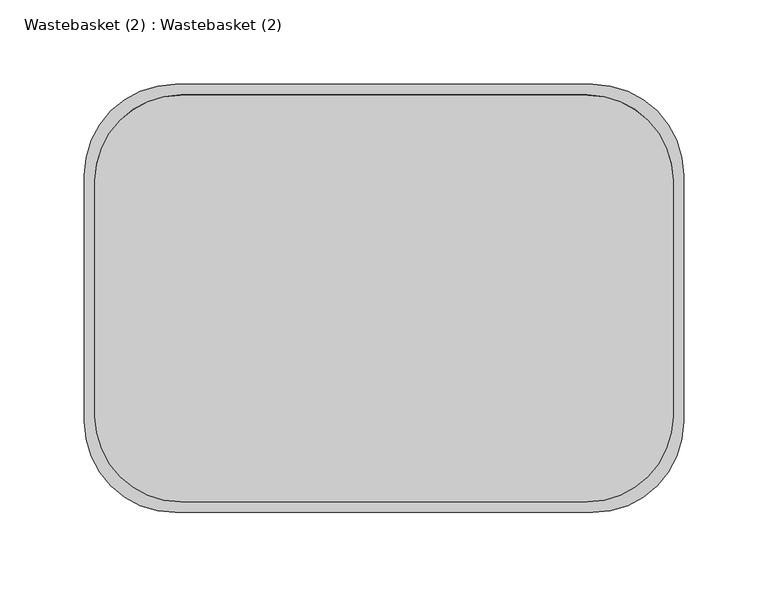
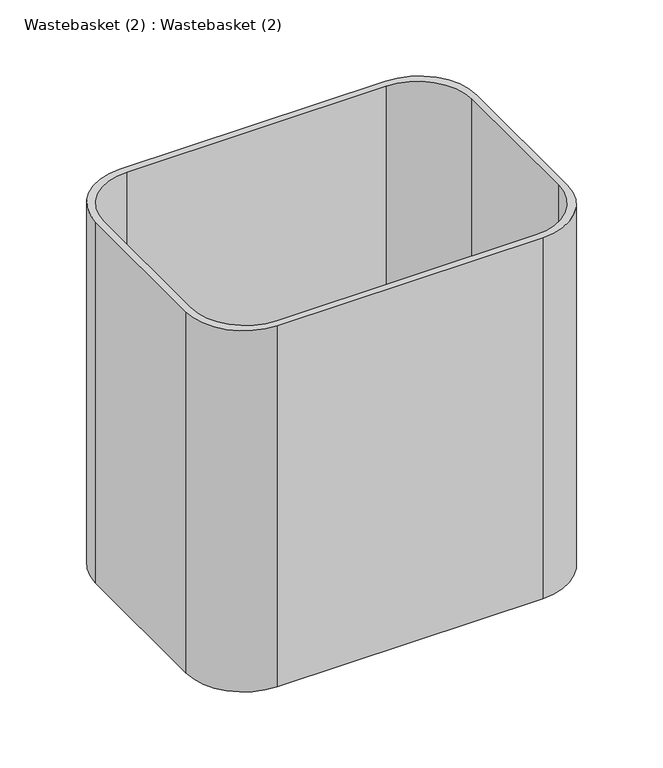
"""IFC4 building model written with IfcOpenShell, lengths in millimetres: furniture geometry, Wastebasket (2) : Wastebasket (2)."""

from ifc_helpers import new_model, si_unit, frame, origin, place, context, project, spatial, polyline, circle_curve, source, transform, mapped, element, save
from ifc_brep_helpers import plane_surface, cylinder_surface, revolved_surface, advanced_brep


def wastebasket_2_wastebasket_2_e1224e57(model_context):
    return source(origin(), model_context, "Body", "AdvancedBrep", [
        advanced_brep(
        [(178.3203994, 170.9615385, 355.6), (-69.3296006, 170.9615385, 355.6), (-123.3046006, 116.9865385, 355.6), (-123.3046006, -29.0634615, 355.6), (-69.3296006, -83.0384615, 355.6), (178.3203994, -83.0384615, 355.6), (232.2953994, -29.0634615, 355.6), (232.2953994, 116.9865385, 355.6), (-66.1546006, 164.6115385, 355.6), (175.1453994, 164.6115385, 355.6), (225.9453994, 113.8115385, 355.6), (225.9453994, -25.8884615, 355.6), (175.1453994, -76.6884615, 355.6), (-66.1546006, -76.6884615, 355.6), (-116.9546006, -25.8884615, 355.6), (-116.9546006, 113.8115385, 355.6), (178.3203994, 170.9615385, 0.0), (232.2953994, 116.9865385, 0.0), (232.2953994, -29.0634615, 0.0), (178.3203994, -83.0384615, 0.0), (-69.3296006, -83.0384615, 0.0), (-123.3046006, -29.0634615, 0.0), (-123.3046006, 116.9865385, 0.0), (-69.3296006, 170.9615385, 0.0), (175.1453994, 164.6115385, 12.7), (-66.1546006, 164.6115385, 12.7), (-116.9546006, 113.8115385, 12.7), (-116.9546006, -25.8884615, 12.7), (-66.1546006, -76.6884615, 12.7), (175.1453994, -76.6884615, 12.7), (225.9453994, -25.8884615, 12.7), (225.9453994, 113.8115385, 12.7)],
        [
            (0, 1),
            (1, 2, circle_curve(frame((-69.3296006, 116.9865385, 355.6), z_axis=(0.0, 0.0, 1.0), x_axis=(1.0, 0.0, 0.0)), 53.975)),
            (2, 3),
            (3, 4, circle_curve(frame((-69.3296006, -29.0634615, 355.6), z_axis=(0.0, 0.0, 1.0), x_axis=(1.0, 0.0, 0.0)), 53.975)),
            (4, 5),
            (5, 6, circle_curve(frame((178.3203994, -29.0634615, 355.6), z_axis=(0.0, 0.0, 1.0), x_axis=(1.0, 0.0, 0.0)), 53.975)),
            (6, 7),
            (7, 0, circle_curve(frame((178.3203994, 116.9865385, 355.6), z_axis=(0.0, 0.0, 1.0), x_axis=(1.0, 0.0, 0.0)), 53.975)),
            (8, 9),
            (9, 10, circle_curve(frame((175.1453994, 113.8115385, 355.6), z_axis=(0.0, 0.0, -1.0), x_axis=(1.0, 0.0, 0.0)), 50.8)),
            (10, 11),
            (11, 12, circle_curve(frame((175.1453994, -25.8884615, 355.6), z_axis=(0.0, 0.0, -1.0), x_axis=(1.0, 0.0, 0.0)), 50.8)),
            (12, 13),
            (13, 14, circle_curve(frame((-66.1546006, -25.8884615, 355.6), z_axis=(0.0, 0.0, -1.0), x_axis=(1.0, 0.0, 0.0)), 50.8)),
            (14, 15),
            (15, 8, circle_curve(frame((-66.1546006, 113.8115385, 355.6), z_axis=(0.0, 0.0, -1.0), x_axis=(1.0, 0.0, 0.0)), 50.8)),
            (16, 17, circle_curve(frame((178.3203994, 116.9865385, 0.0), z_axis=(0.0, 0.0, -1.0), x_axis=(1.0, 0.0, 0.0)), 53.975)),
            (17, 18),
            (18, 19, circle_curve(frame((178.3203994, -29.0634615, 0.0), z_axis=(0.0, 0.0, -1.0), x_axis=(1.0, 0.0, 0.0)), 53.975)),
            (19, 20),
            (20, 21, circle_curve(frame((-69.3296006, -29.0634615, 0.0), z_axis=(0.0, 0.0, -1.0), x_axis=(1.0, 0.0, 0.0)), 53.975)),
            (21, 22),
            (22, 23, circle_curve(frame((-69.3296006, 116.9865385, 0.0), z_axis=(0.0, 0.0, -1.0), x_axis=(1.0, 0.0, 0.0)), 53.975)),
            (23, 16),
            (0, 16),
            (23, 1),
            (22, 2),
            (21, 3),
            (20, 4),
            (19, 5),
            (18, 6),
            (17, 7),
            (24, 25),
            (25, 26, circle_curve(frame((-66.1546006, 113.8115385, 12.7), z_axis=(0.0, 0.0, 1.0), x_axis=(1.0, 0.0, 0.0)), 50.8)),
            (26, 27),
            (27, 28, circle_curve(frame((-66.1546006, -25.8884615, 12.7), z_axis=(0.0, 0.0, 1.0), x_axis=(1.0, 0.0, 0.0)), 50.8)),
            (28, 29),
            (29, 30, circle_curve(frame((175.1453994, -25.8884615, 12.7), z_axis=(0.0, 0.0, 1.0), x_axis=(1.0, 0.0, 0.0)), 50.8)),
            (30, 31),
            (31, 24, circle_curve(frame((175.1453994, 113.8115385, 12.7), z_axis=(0.0, 0.0, 1.0), x_axis=(1.0, 0.0, 0.0)), 50.8)),
            (24, 9),
            (8, 25),
            (15, 26),
            (14, 27),
            (13, 28),
            (12, 29),
            (11, 30),
            (10, 31),
        ],
        [
            plane_surface(frame((-123.3046006, 170.9615385, 355.6), z_axis=(0.0, 0.0, 1.0), x_axis=(-1.0, 0.0, 0.0))),
            plane_surface(frame((-123.3046006, 170.9615385, 0.0), z_axis=(0.0, 0.0, -1.0), x_axis=(1.0, 0.0, 0.0))),
            plane_surface(frame((178.3203994, 170.9615385, 355.6), z_axis=(0.0, 1.0, 0.0), x_axis=(0.0, 0.0, -1.0))),
            cylinder_surface(frame((-69.3296006, 116.9865385, 0.0), z_axis=(0.0, 0.0, 1.0), x_axis=(1.0, 0.0, 0.0)), 53.975),
            plane_surface(frame((-123.3046006, 116.9865385, 355.6), z_axis=(-1.0, 0.0, 0.0), x_axis=(0.0, 0.0, -1.0))),
            cylinder_surface(frame((-69.3296006, -29.0634615, 0.0), z_axis=(0.0, 0.0, 1.0), x_axis=(1.0, 0.0, 0.0)), 53.975),
            plane_surface(frame((-69.3296006, -83.0384615, 355.6), z_axis=(0.0, -1.0, 0.0), x_axis=(0.0, 0.0, -1.0))),
            cylinder_surface(frame((178.3203994, -29.0634615, 0.0), z_axis=(0.0, 0.0, 1.0), x_axis=(1.0, 0.0, 0.0)), 53.975),
            plane_surface(frame((232.2953994, -29.0634615, 355.6), z_axis=(1.0, 0.0, 0.0), x_axis=(0.0, 0.0, -1.0))),
            cylinder_surface(frame((178.3203994, 116.9865385, 0.0), z_axis=(0.0, 0.0, 1.0), x_axis=(1.0, 0.0, 0.0)), 53.975),
            plane_surface(frame((-66.1546006, 164.6115385, 12.7), z_axis=(0.0, 0.0, 1.0), x_axis=(1.0, 0.0, 0.0))),
            plane_surface(frame((175.1453994, 164.6115385, 355.6), z_axis=(0.0, -1.0, 0.0), x_axis=(0.0, 0.0, -1.0))),
            revolved_surface(polyline([(-15.354600599999998, 113.8115385, 355.6), (-15.354600599999998, 113.8115385, 12.7)]), (-66.1546006, 113.8115385, 12.7), (0.0, 0.0, 1.0)),
            plane_surface(frame((-116.9546006, 113.8115385, 355.6), z_axis=(1.0, 0.0, 0.0), x_axis=(0.0, 0.0, -1.0))),
            revolved_surface(polyline([(-15.354600599999998, -25.8884615, 355.6), (-15.354600599999998, -25.8884615, 12.7)]), (-66.1546006, -25.8884615, 12.7), (0.0, 0.0, 1.0)),
            plane_surface(frame((-66.1546006, -76.6884615, 355.6), z_axis=(0.0, 1.0, 0.0), x_axis=(0.0, 0.0, -1.0))),
            revolved_surface(polyline([(225.94539939999999, -25.8884615, 355.6), (225.94539939999999, -25.8884615, 12.7)]), (175.1453994, -25.8884615, 12.7), (0.0, 0.0, 1.0)),
            plane_surface(frame((225.9453994, -25.8884615, 355.6), z_axis=(-1.0, 0.0, 0.0), x_axis=(0.0, 0.0, -1.0))),
            revolved_surface(polyline([(225.94539939999999, 113.8115385, 355.6), (225.94539939999999, 113.8115385, 12.7)]), (175.1453994, 113.8115385, 12.7), (0.0, 0.0, 1.0)),
        ],
        [
            (0, [[1, 2, 3, 4, 5, 6, 7, 8], [9, 10, 11, 12, 13, 14, 15, 16]]),
            (1, [[17, 18, 19, 20, 21, 22, 23, 24]]),
            (2, [[-1, 25, -24, 26]]),
            (3, [[-2, -26, -23, 27]]),
            (4, [[-3, -27, -22, 28]]),
            (5, [[-4, -28, -21, 29]]),
            (6, [[-5, -29, -20, 30]]),
            (7, [[-6, -30, -19, 31]]),
            (8, [[-7, -31, -18, 32]]),
            (9, [[-8, -32, -17, -25]]),
            (10, [[33, 34, 35, 36, 37, 38, 39, 40]]),
            (11, [[-33, 41, -9, 42]]),
            (12, [[-34, -42, -16, 43]]),
            (13, [[-35, -43, -15, 44]]),
            (14, [[-36, -44, -14, 45]]),
            (15, [[-37, -45, -13, 46]]),
            (16, [[-38, -46, -12, 47]]),
            (17, [[-39, -47, -11, 48]]),
            (18, [[-40, -48, -10, -41]]),
        ],
    ),
    ])


if __name__ == "__main__":
    model = new_model("IFC4")
    model_context = context("Model", 3, world=origin())
    ifc_project = project(units=[si_unit("LENGTHUNIT", "METRE", prefix="MILLI")], contexts=[model_context])
    site = spatial("IfcSite", under=ifc_project)
    building = spatial("IfcBuilding", under=site)
    placement = place(None, origin())
    wastebasket_2_wastebasket_2_shape = wastebasket_2_wastebasket_2_e1224e57(model_context)
    element("IfcFurniture", 1, ObjectType="Wastebasket (2) : Wastebasket (2)", at=placement, inside=building, context=model_context, shape_type="MappedRepresentation", body=[
        mapped(wastebasket_2_wastebasket_2_shape, transform((0.0, 0.0, 0.0), x_axis=(1.0, 0.0, 0.0), y_axis=(0.0, 1.0, 0.0), z_axis=(0.0, 0.0, 1.0))),
    ])
    save(model, "model.ifc")

# Revit data of these elements
# Type "Wastebasket (2) : Wastebasket (2)"
#   Keynote = "N"
#   Material Bin = Metal - Chrome
#   Assembly Code = ""
# Element 1 (IfcFurniture, "Wastebasket (2) : Wastebasket (2)")
#   Materials on its faces: "Metal - Chrome"
# Materials
#   "Metal - Chrome": class "Metal", colour RGB 206 206 206, transparency 0
